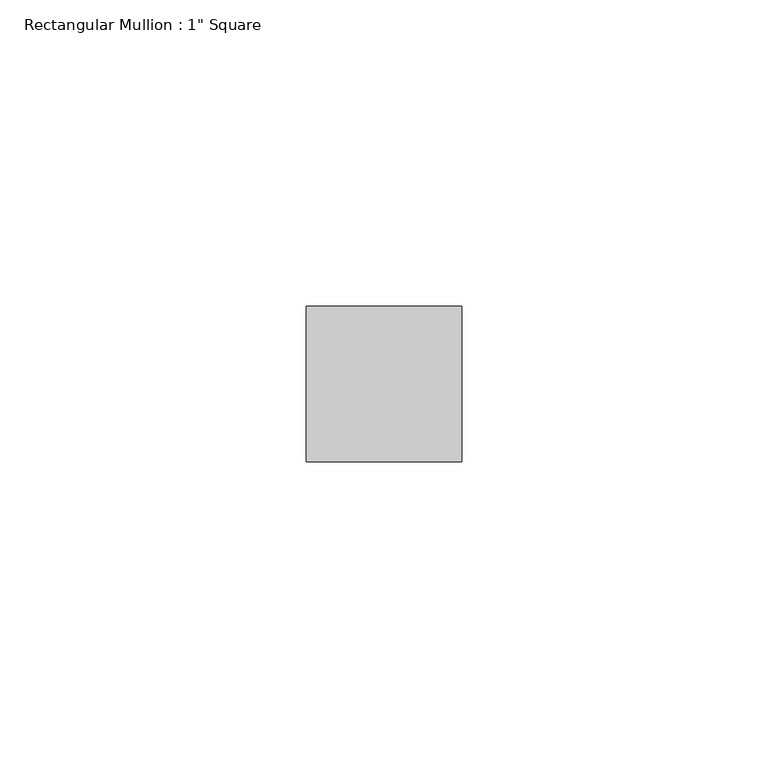
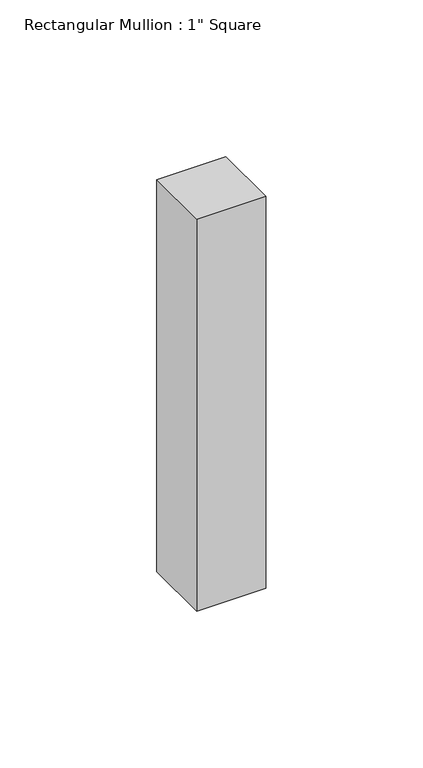
"""IFC4 building model written with IfcOpenShell, lengths in millimetres: member geometry."""

from ifc_helpers import new_model, si_unit, frame, origin, place, context, project, spatial, polyline, outline, extrude, source, transform, mapped, element, save


def member_e752087b(model_context):
    return source(origin(), model_context, "Body", "SweptSolid", [
        extrude(outline(polyline([(0.0, 12.7), (0.0, -12.7), (-25.4, -12.7), (-25.4, 12.7), (0.0, 12.7)])), frame((0.0, 0.0, -152.4), z_axis=(0.0, 0.0, 1.0), x_axis=(1.0, 0.0, 0.0)), (0.0, 0.0, 1.0), 152.4),
    ])


if __name__ == "__main__":
    model = new_model("IFC4")
    model_context = context("Model", 3, world=origin())
    ifc_project = project(units=[si_unit("LENGTHUNIT", "METRE", prefix="MILLI")], contexts=[model_context])
    site = spatial("IfcSite", under=ifc_project)
    building = spatial("IfcBuilding", under=site)
    placement = place(None, origin())
    member_shape = member_e752087b(model_context)
    element("IfcMember", 1, ObjectType="Rectangular Mullion : 1\" Square", at=placement, inside=building, context=model_context, shape_type="MappedRepresentation", body=[
        mapped(member_shape, transform((0.0, 0.0, 0.0), x_axis=(1.0, 0.0, 0.0), y_axis=(0.0, 1.0, 0.0), z_axis=(0.0, 0.0, 1.0))),
    ])
    save(model, "model.ifc")

# Revit data of these elements
# Type "Rectangular Mullion : 1\" Square"
#   built-in parameter 1007304 = 0.0833333 (stored number, unit not read)
#   built-in parameter 1007301 = 0.0416667 (stored number, unit not read)
#   built-in parameter 1007300 = 0.0416667 (stored number, unit not read)
# Element 1 (IfcMember, "Rectangular Mullion : 1\" Square")
#   Materials on its faces: "Metal - Aluminum"
# Materials
#   "Metal - Aluminum": class "Metal", colour RGB 247 247 247, transparency 0
